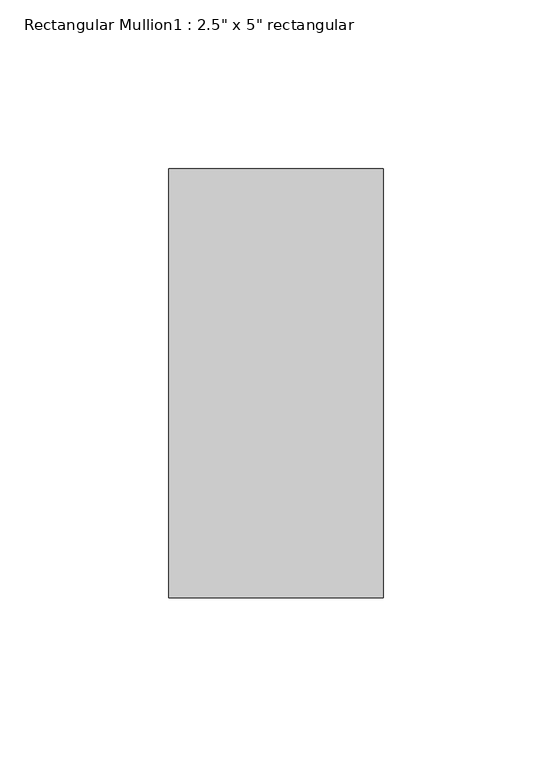
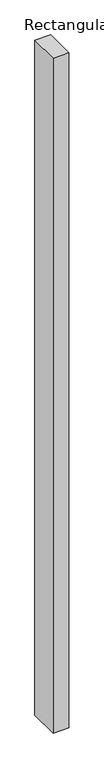
"""IFC4 building model written with IfcOpenShell, lengths in millimetres: member geometry."""

from ifc_helpers import new_model, si_unit, frame, origin, place, context, project, spatial, polyline, outline, extrude, source, transform, mapped, element, save


def member_e54787da(model_context):
    return source(origin(), model_context, "Body", "SweptSolid", [
        extrude(outline(polyline([(31.75, 63.5), (31.75, -63.5), (-31.75, -63.5), (-31.75, 63.5), (31.75, 63.5)])), frame((0.0, 0.0, -2884.17), z_axis=(0.0, 0.0, 1.0), x_axis=(1.0, 0.0, 0.0)), (0.0, 0.0, 1.0), 2884.17),
    ])


if __name__ == "__main__":
    model = new_model("IFC4")
    model_context = context("Model", 3, world=origin())
    ifc_project = project(units=[si_unit("LENGTHUNIT", "METRE", prefix="MILLI")], contexts=[model_context])
    site = spatial("IfcSite", under=ifc_project)
    building = spatial("IfcBuilding", under=site)
    placement = place(None, origin())
    member_shape = member_e54787da(model_context)
    element("IfcMember", 1, ObjectType="Rectangular Mullion1 : 2.5\" x 5\" rectangular", at=placement, inside=building, context=model_context, shape_type="MappedRepresentation", body=[
        mapped(member_shape, transform((0.0, 0.0, 0.0), x_axis=(1.0, 0.0, 0.0), y_axis=(0.0, 1.0, 0.0), z_axis=(0.0, 0.0, 1.0))),
    ])
    save(model, "model.ifc")

# Revit data of these elements
# Type "Rectangular Mullion1 : 2.5\" x 5\" rectangular"
#   built-in parameter 1007304 = 0.416667 (stored number, unit not read)
#   built-in parameter 1007301 = 0.104167 (stored number, unit not read)
#   built-in parameter 1007300 = 0.104167 (stored number, unit not read)
# Element 1 (IfcMember, "Rectangular Mullion1 : 2.5\" x 5\" rectangular")
#   Materials on its faces: "support-frame"
# Materials
#   "support-frame": class "Unassigned", colour RGB 233 233 233, transparency 0, Cost = 0
